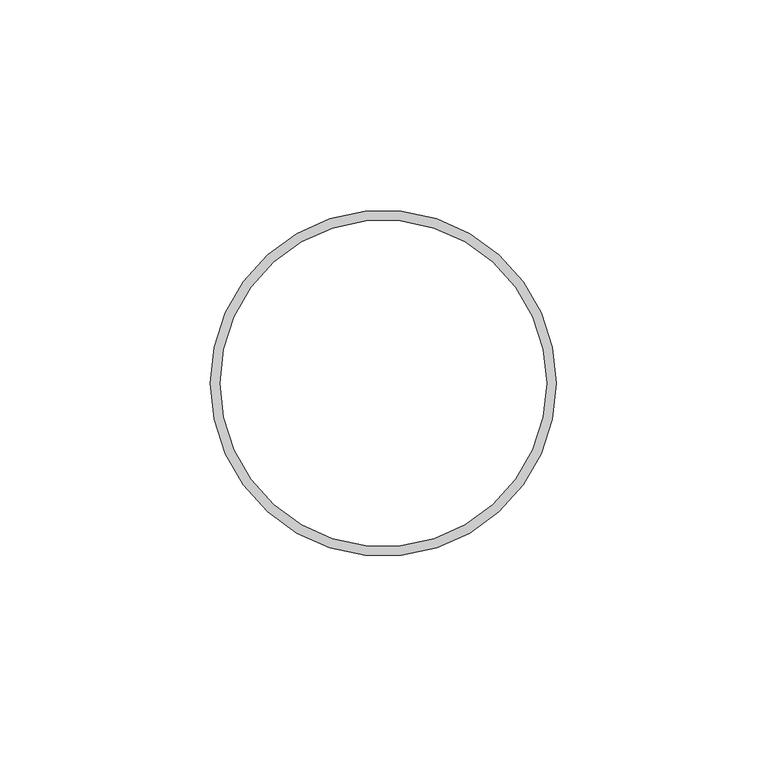
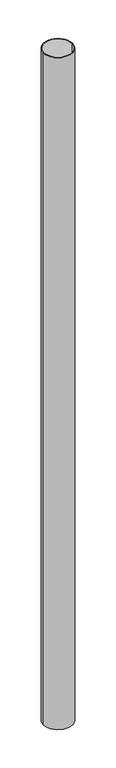
"""IFC4 building model written with IfcOpenShell, lengths in millimetres: proxy geometry, TN_ПВС 125-82_Водосточная труба : TN_ПВС 125-82_Водосточная труба."""

from ifc_helpers import new_model, si_unit, point, origin, origin_with_axes, origin_2d, place, context, project, spatial, circle_curve, trimmed, segment, composite_curve, outline, extrude, source, transform, mapped, element, save


def generic_models_a5ae73a3(model_context):
    return source(origin(), model_context, "Body", "SweptSolid", [
        extrude(outline(composite_curve([segment(trimmed(circle_curve(origin_2d(), 41.1), [point((-41.1, 0.0))], [point((41.1, 0.0))], False, "CARTESIAN"), True, "CONTINUOUS"), segment(trimmed(circle_curve(origin_2d(), 41.1), [point((41.1, 0.0))], [point((-41.1, 0.0))], False, "CARTESIAN"), True, "CONTINUOUS")], self_intersect=False), holes=[composite_curve([segment(trimmed(circle_curve(origin_2d(), 38.8), [point((-38.8, 0.0))], [point((38.8, 0.0))], True, "CARTESIAN"), True, "CONTINUOUS"), segment(trimmed(circle_curve(origin_2d(), 38.8), [point((38.8, 0.0))], [point((-38.8, 0.0))], True, "CARTESIAN"), True, "CONTINUOUS")], self_intersect=False)]), origin_with_axes(), (0.0, 0.0, 1.0), 2000.0),
    ])


if __name__ == "__main__":
    model = new_model("IFC4")
    model_context = context("Model", 3, world=origin())
    ifc_project = project(units=[si_unit("LENGTHUNIT", "METRE", prefix="MILLI")], contexts=[model_context])
    site = spatial("IfcSite", under=ifc_project)
    building = spatial("IfcBuilding", under=site)
    placement = place(None, origin())
    generic_models_shape = generic_models_a5ae73a3(model_context)
    element("IfcBuildingElementProxy", 1, Name="TN_ПВС 125-82_Водосточная труба : TN_ПВС 125-82_Водосточная труба", ObjectType="TN_ПВС 125-82_Водосточная труба : TN_ПВС 125-82_Водосточная труба", at=placement, inside=building, context=model_context, shape_type="MappedRepresentation", body=[
        mapped(generic_models_shape, transform((0.0, 0.0, 0.0), x_axis=(1.0, 0.0, 0.0), y_axis=(0.0, 1.0, 0.0), z_axis=(0.0, 0.0, 1.0))),
    ])
    save(model, "model.ifc")

# Revit data of these elements
# Type "TN_ПВС 125-82_Водосточная труба : TN_ПВС 125-82_Водосточная труба"
#   Description = "Организует вертикальный сток дождевой воды"
#   Manufacturer = "ТехноНИКОЛЬ"
#   Model = "Комплектующие к водосточным системам"
#   URL = "https://tn-vodostok.ru/catalog/pvh/"
#   ADSK_Обозначение = "ТехноНИКОЛЬ"
#   ADSK_Наименование краткое = "Труба"
#   ADSK_Наименование = "Водосточная труба"
#   ADSK_Масса_Текст = ""
#   ADSK_Марка = ""
#   ADSK_Код изделия = ""
#   ADSK_Завод-изготовитель = "ТехноНИКОЛЬ"
#   ADSK_Единица измерения = "п.м."
#   ADSK_Группирование = "Комплектующие к водосточным системам"
#   ADSK_URL страницы изделия = "https://tn-vodostok.ru/catalog/pvh/"
#   ADSK_URL документации изделия = "https://tn-vodostok.ru/upload/iblock/c42/c427963cb77eb5c3c51f0cfb870e9e52.pdf"
#   ADSK_Размер_Диаметр = 82.2 mm
#   ADSK_Размер_Высота [instance default] = 500 mm
#   ADSK_Количество [instance default] = 0.5
#   ADSK_Материал [instance default] = TN_Пластик_Коричневый_RAL8019
#   Default Elevation = 0
# Element 1 (IfcBuildingElementProxy, "TN_ПВС 125-82_Водосточная труба : TN_ПВС 125-82_Водосточная труба")
#   ADSK_Размер_Высота = 2000 mm
#   ADSK_Количество = 2
#   Materials on its faces: "TN_Пластик_Коричневый_RAL8019"
# Materials
#   "TN_Пластик_Коричневый_RAL8019": class "Типовые", colour RGB 61 54 53, transparency 0, Cost = 0
